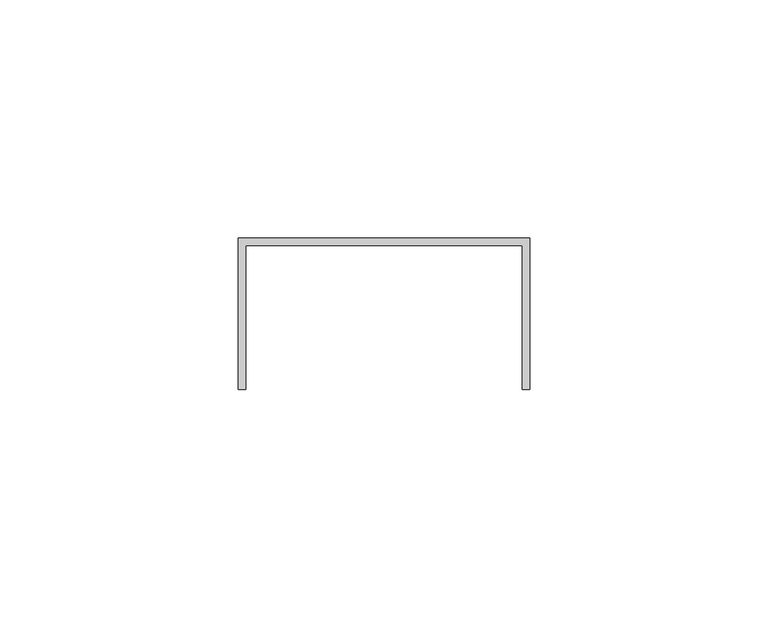
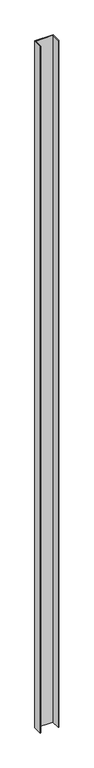
"""IFC4 building model written with IfcOpenShell, lengths in millimetres: proxy geometry, Generic Models 7:Generic Models 1:3:Generic Models 1:3 : Generic Models 7:Generic Models 1:305549:3:Generic Models 1:3:Generic Models 1:3 : Generic Models 7:Generic Models 1:305549:3 : Generic Models 7:Generic Models 1:3:Generic Models 1:3 : Generic Models 7:Generic Models 1:305549:301244:66 : Generic Models 7:Generic Models 1:3:Generic Models 1:3 : Generic Models 7:Generic Models 1:305549:3:Generic Models 1:3:Generic Models 1:3 : Generic Models 7:Generic Models 1:305549:3 : Generic Models 7:Generic Models 1:3:Generic Models 1:3 : Generic Models 7:Generic Models 1:305549:301244:308848."""

from ifc_helpers import new_model, si_unit, frame, origin, place, context, project, spatial, polyline, outline, extrude, source, transform, mapped, element, save


def generic_models_5d313a6e(model_context):
    return source(origin(), model_context, "Body", "SweptSolid", [
        extrude(outline(polyline([(560350.5804739, -530645.4413841), (560350.5804739, -530677.1913841), (560348.9929739, -530677.1913841), (560348.9929739, -530647.0288841), (560291.0492239, -530647.0288841), (560291.0492239, -530677.1913841), (560289.4617239, -530677.1913841), (560289.4617239, -530645.4413841), (560350.5804739, -530645.4413841)])), frame((0.0, 0.0, 50.8), z_axis=(0.0, 0.0, 1.0), x_axis=(1.0, 0.0, 0.0)), (0.0, 0.0, 1.0), 2430.9324376),
    ])


if __name__ == "__main__":
    model = new_model("IFC4")
    model_context = context("Model", 3, world=origin())
    ifc_project = project(units=[si_unit("LENGTHUNIT", "METRE", prefix="MILLI")], contexts=[model_context])
    site = spatial("IfcSite", under=ifc_project)
    building = spatial("IfcBuilding", under=site)
    placement = place(None, origin())
    generic_models_shape = generic_models_5d313a6e(model_context)
    element("IfcBuildingElementProxy", 1, Name="Generic Models 7:Generic Models 1:3:Generic Models 1:3 : Generic Models 7:Generic Models 1:305549:3:Generic Models 1:3:Generic Models 1:3 : Generic Models 7:Generic Models 1:305549:3 : Generic Models 7:Generic Models 1:3:Generic Models 1:3 : Generic Models 7:Generic Models 1:305549:301244:66 : Generic Models 7:Generic Models 1:3:Generic Models 1:3 : Generic Models 7:Generic Models 1:305549:3:Generic Models 1:3:Generic Models 1:3 : Generic Models 7:Generic Models 1:305549:3 : Generic Models 7:Generic Models 1:3:Generic Models 1:3 : Generic Models 7:Generic Models 1:305549:301244:308848", ObjectType="Generic Models 7:Generic Models 1:3:Generic Models 1:3 : Generic Models 7:Generic Models 1:305549:3:Generic Models 1:3:Generic Models 1:3 : Generic Models 7:Generic Models 1:305549:3 : Generic Models 7:Generic Models 1:3:Generic Models 1:3 : Generic Models 7:Generic Models 1:305549:301244:66 : Generic Models 7:Generic Models 1:3:Generic Models 1:3 : Generic Models 7:Generic Models 1:305549:3:Generic Models 1:3:Generic Models 1:3 : Generic Models 7:Generic Models 1:305549:3 : Generic Models 7:Generic Models 1:3:Generic Models 1:3 : Generic Models 7:Generic Models 1:305549:301244:308848", at=placement, inside=building, context=model_context, shape_type="MappedRepresentation", body=[
        mapped(generic_models_shape, transform((0.0, 0.0, 0.0), x_axis=(1.0, 0.0, 0.0), y_axis=(0.0, 1.0, 0.0), z_axis=(0.0, 0.0, 1.0))),
    ])
    save(model, "model.ifc")

# Revit data of these elements
# Type "Generic Models 7:Generic Models 1:3:Generic Models 1:3 : Generic Models 7:Generic Models 1:305549:3:Generic Models 1:3:Generic Models 1:3 : Generic Models 7:Generic Models 1:305549:3 : Generic Models 7:Generic Models 1:3:Generic Models 1:3 : Generic Models 7:Generic Models 1:305549:301244:66 : Generic Models 7:Generic Models 1:3:Generic Models 1:3 : Generic Models 7:Generic Models 1:305549:3:Generic Models 1:3:Generic Models 1:3 : Generic Models 7:Generic Models 1:305549:3 : Generic Models 7:Generic Models 1:3:Generic Models 1:3 : Generic Models 7:Generic Models 1:305549:301244:308848"
#   NameOverride = "Generic Models 7:Generic Models 1:3:Generic Models 1:3 : Generic Models 7:Generic Models 1:305549:3:Generic Models 1:3:Generic Models 1:3 : Generic Models 7:Generic Models 1:305549:3 : Generic Models 7:Generic Models 1:3:Generic Models 1:3 : Generic Models 7:Generic Models 1:305549:301244:308848"
#   ObjectTypeOverride = "Generic Models 1:3:Generic Models 1:3 : Generic Models 7:Generic Models 1:305549:3 : Generic Models 7:Generic Models 1:3:Generic Models 1:3 : Generic Models 7:Generic Models 1:305549:301244"
#   Reference = "Generic Models 1"
#   Tag = "308848"
# Element 1 (IfcBuildingElementProxy, "Generic Models 7:Generic Models 1:3:Generic Models 1:3 : Generic Models 7:Generic Models 1:305549:3:Generic Models 1:3:Generic Models 1:3 : Generic Models 7:Generic Models 1:305549:3 : Generic Models 7:Generic Models 1:3:Generic Models 1:3 : Generic Models 7:Generic Models 1:305549:301244:66 : Generic Models 7:Generic Models 1:3:Generic Models 1:3 : Generic Models 7:Generic Models 1:305549:3:Generic Models 1:3:Generic Models 1:3 : Generic Models 7:Generic Models 1:305549:3 : Generic Models 7:Generic Models 1:3:Generic Models 1:3 : Generic Models 7:Generic Models 1:305549:301244:308848")
#   Materials on its faces: "GALVANIZED U-CHANNEL (250T125-33)"
# Materials
#   "GALVANIZED U-CHANNEL (250T125-33)": class "Unassigned", colour RGB 202 201 200, transparency 0, Keynote = "M05451300.02", Cost = 0
